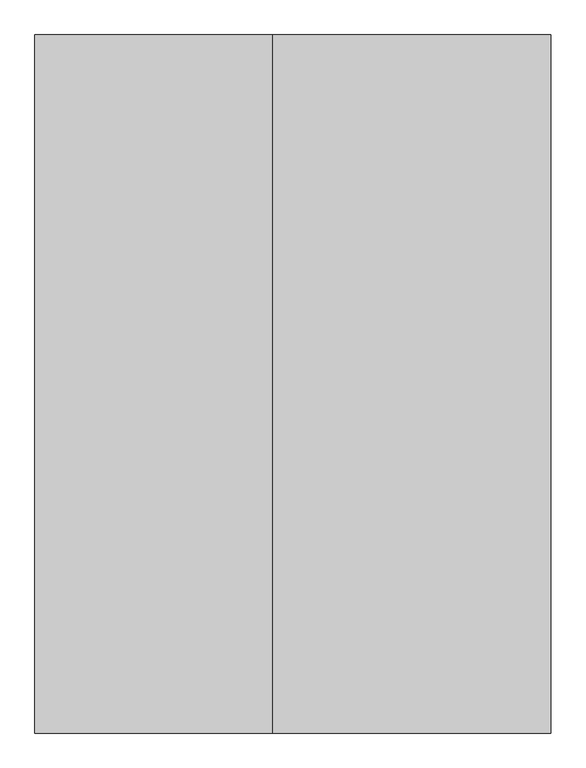
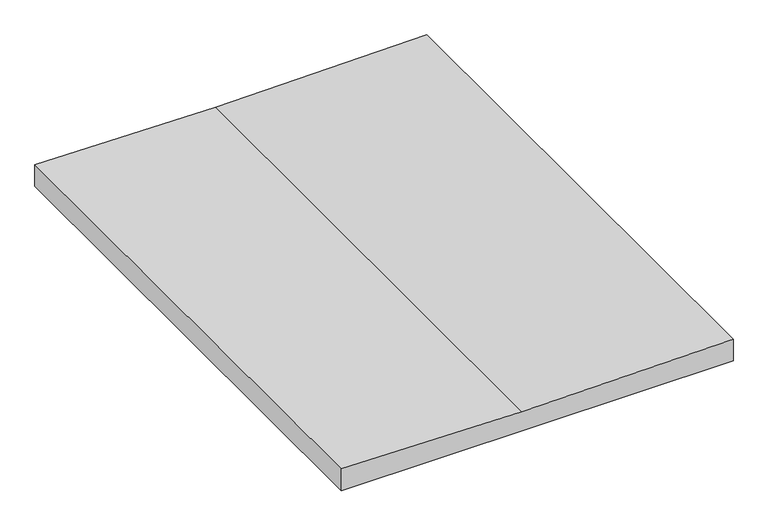
"""IFC4 building model written with IfcOpenShell, lengths in millimetres: proxy geometry, FIRESTONE INSULATION001 4237 : FIRESTONE INSULATION001 4237."""

from ifc_helpers import new_model, si_unit, frame, origin, place, context, project, spatial, polyline, outline, extrude, source, transform, mapped, element, save


def generic_models_f580233c(model_context):
    return source(origin(), model_context, "Body", "SweptSolid", [
        extrude(outline(polyline([(40131.746, -2567.3737014), (40131.746, -1090.0815411), (40218.4000089, -1090.0815411), (40208.6021556, -1886.5629484), (40218.4000089, -2567.3737014), (40131.746, -2567.3737014)])), frame((0.0, -1052.6406573, 0.0), z_axis=(0.0, 1.0, 0.0), x_axis=(0.0, 0.0, 1.0)), (0.0, 0.0, 1.0), 2000.0),
    ])


if __name__ == "__main__":
    model = new_model("IFC4")
    model_context = context("Model", 3, world=origin())
    ifc_project = project(units=[si_unit("LENGTHUNIT", "METRE", prefix="MILLI")], contexts=[model_context])
    site = spatial("IfcSite", under=ifc_project)
    building = spatial("IfcBuilding", under=site)
    placement = place(None, origin())
    generic_models_shape = generic_models_f580233c(model_context)
    element("IfcBuildingElementProxy", 1, Name="FIRESTONE INSULATION001 4237 : FIRESTONE INSULATION001 4237", ObjectType="FIRESTONE INSULATION001 4237 : FIRESTONE INSULATION001 4237", at=placement, inside=building, context=model_context, shape_type="MappedRepresentation", body=[
        mapped(generic_models_shape, transform((0.0, 0.0, 0.0), x_axis=(1.0, 0.0, 0.0), y_axis=(0.0, 1.0, 0.0), z_axis=(0.0, 0.0, 1.0))),
    ])
    save(model, "model.ifc")

# Revit data of these elements
# Type "FIRESTONE INSULATION001 4237 : FIRESTONE INSULATION001 4237"
#   NameOverride = "FIRESTONE INSULATION001"
# Element 1 (IfcBuildingElementProxy, "FIRESTONE INSULATION001 4237 : FIRESTONE INSULATION001 4237")
#   Materials on its faces: "TAPERED 2X SLEEPERS - SLOPED TO DRAIN"
# Materials
#   "TAPERED 2X SLEEPERS - SLOPED TO DRAIN": class "Unassigned", colour RGB 234 198 178, transparency 0
